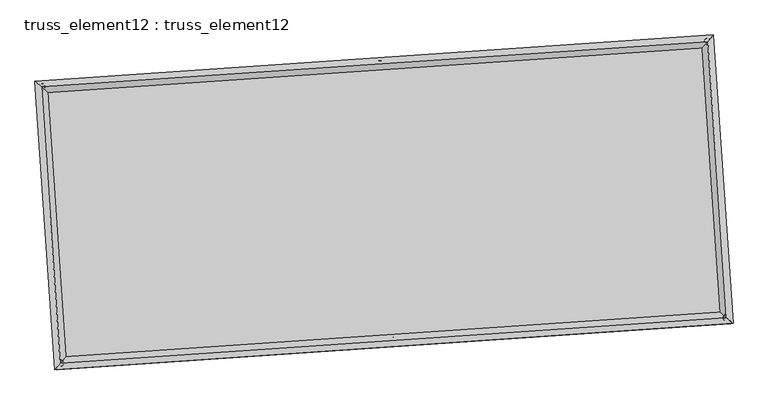
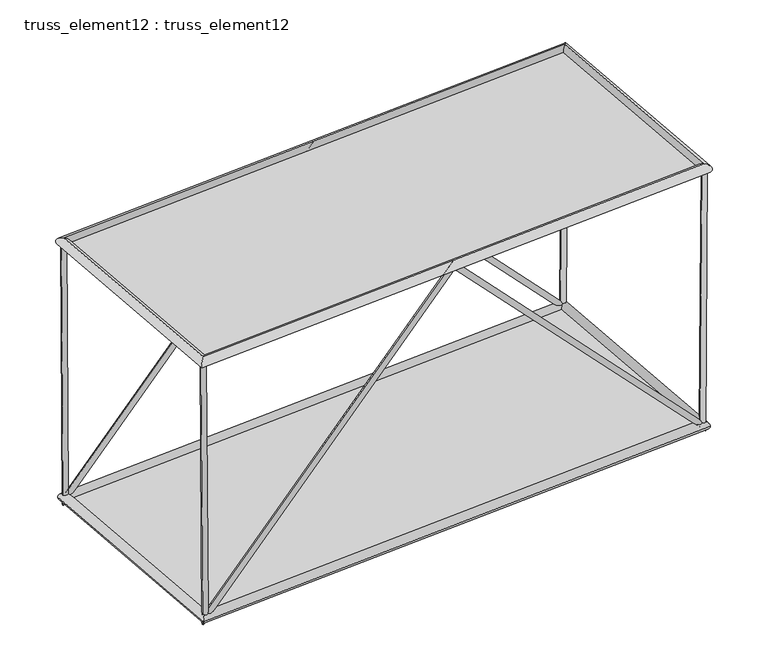
"""IFC4 building model written with IfcOpenShell, lengths in millimetres: plate geometry, truss_element12 : truss_element12."""

from ifc_helpers import new_model, si_unit, frame, origin, origin_with_axes, place, context, project, spatial, polyline, circle_curve, ellipse_curve, outline, extrude, source, transform, mapped, element, save
from ifc_brep_helpers import plane_surface, cylinder_surface, advanced_brep


def truss_element12_truss_element12_8e9da1f8(model_context):
    return source(origin(), model_context, "Body", "SolidModel", [
        advanced_brep(
        [(-3698.7518615, 2273.9185866, 5000.223301), (-3797.8529392, 2260.5574847, 4999.5470243), (-3665.7745625, 2276.1671833, 123.3293266), (-3763.2123204, 2262.9194968, -123.3293266), (1063.9844604, 2598.6714715, 5072.0064402), (1064.4287053, 2592.0979868, 4927.7602832), (5793.2263236, 2921.1404966, 123.3255902), (5891.5346534, 2921.2399919, -123.3255902), (5826.7168605, 2923.424089, 5000.224961), (5926.7142716, 2923.6387563, 4999.5381605)],
        [
            (0, 1, circle_curve(frame((-3748.3024003, 2267.2380357, 4999.8851627), z_axis=(-0.0067617917796413095, -0.00046106087747684727, 0.9999770325336459), x_axis=(-0.13361106793445865, 0.9910337446995272, -0.0004465335886331621)), 50.0)),
            (1, 0, circle_curve(frame((-3748.3024003, 2267.2380357, 4999.8851627), z_axis=(-0.0067617917796413095, -0.00046106087747684727, 0.9999770325336459), x_axis=(-0.13361106793445865, 0.9910337446995272, -0.0004465335886331621)), 50.0)),
            (0, 2),
            (2, 3, ellipse_curve(frame((-3714.4934414, 2269.54334, 0.0), z_axis=(-0.9270371329382548, -0.06321113809700207, 0.3696031739231987), x_axis=(0.3687469497597502, 0.025143452765731104, 0.9291896974385251)), 133.0168379, 50.0)),
            (3, 1),
            (3, 2, ellipse_curve(frame((-3714.4934414, 2269.54334, 0.0), z_axis=(-0.9270371329382548, -0.06321113809700207, 0.3696031739231987), x_axis=(0.3687469497597502, 0.025143452765731104, 0.9291896974385251)), 133.0168379, 50.0)),
            (2, 4),
            (4, 5, ellipse_curve(frame((1064.2065829, 2595.3847292, 4999.8833617), z_axis=(-0.9976833956976204, -0.06802823820297674, 2.7500260085138387e-05), x_axis=(-2.74365528747556e-05, -1.8707942443931063e-06, -0.9999999996218679)), 72.2801261, 50.0)),
            (5, 3),
            (5, 4, ellipse_curve(frame((1064.2065829, 2595.3847292, 4999.8833617), z_axis=(-0.9976833956976204, -0.06802823820297674, 2.7500260085138387e-05), x_axis=(-2.74365528747556e-05, -1.8707942443931063e-06, -0.9999999996218679)), 72.2801261, 50.0)),
            (4, 6),
            (6, 7, ellipse_curve(frame((5842.3804885, 2921.1902443, 0.0), z_axis=(-0.9270667165570741, -0.0632131552915117, -0.3695286187160294), x_axis=(-0.3686725672674666, -0.0251383809063366, 0.9292193497500056)), 133.0085635, 50.0)),
            (7, 5),
            (7, 6, ellipse_curve(frame((5842.3804885, 2921.1902443, 0.0), z_axis=(-0.9270667165570741, -0.0632131552915117, -0.3695286187160294), x_axis=(-0.3686725672674666, -0.0251383809063366, 0.9292193497500056)), 133.0085635, 50.0)),
            (8, 9, circle_curve(frame((5876.715566, 2923.5314227, 4999.8815607), z_axis=(0.0068670155092968675, 0.0004682356836093084, 0.9999763121461127), x_axis=(-0.00214983747870396, 0.9999975862733836, -0.0004534823281307776)), 50.0)),
            (9, 8, circle_curve(frame((5876.715566, 2923.5314227, 4999.8815607), z_axis=(0.0068670155092968675, 0.0004682356836093084, 0.9999763121461127), x_axis=(-0.00214983747870396, 0.9999975862733836, -0.0004534823281307776)), 50.0)),
            (6, 8),
            (9, 7),
        ],
        [
            plane_surface(frame((-3748.3024003, 2317.2380303, 4999.9082162), z_axis=(-0.006761791779640632, -0.0004610608774721699, 0.9999770325336457), x_axis=(0.9999771388246477, -3.1176689248013658e-06, 0.006761791060906577))),
            cylinder_surface(frame((-3748.3024003, 2267.2380357, 4999.8851627), z_axis=(-0.006761791779641308, -0.00046106087747684716, 0.9999770325336457), x_axis=(-0.13361106793445865, 0.9910337446995272, -0.0004465335886331621)), 50.0),
            cylinder_surface(frame((-3714.4934414, 2269.54334, 0.0), z_axis=(-0.6901703766804573, -0.0470600944026198, -0.7221150868577476), x_axis=(-0.020414252830953418, 0.9987522052200565, -0.045577306298510874)), 50.0),
            cylinder_surface(frame((1064.2065829, 2595.3847292, 4999.8833617), z_axis=(-0.6901307509390454, -0.04705739247394453, 0.7221531336370857), x_axis=(-0.11534910612614199, 0.9922789584550205, -0.045574689503274965)), 50.0),
            plane_surface(frame((5876.715566, 2873.5314282, 4999.9049731), z_axis=(0.006867015509297537, 0.00046823568361033024, 0.9999763121461126), x_axis=(0.9999764217710311, -3.215457516247967e-06, -0.006867014756483772))),
            cylinder_surface(frame((5842.3804885, 2921.1902443, 0.0), z_axis=(-0.0068670155092968675, -0.0004682356836093084, -0.9999763121461127), x_axis=(-0.00214983747870396, 0.9999975862733836, -0.0004534823281307776)), 50.0),
        ],
        [
            (0, [[1, 2]]),
            (1, [[-1, 3, 4, 5]]),
            (1, [[-2, -5, 6, -3]]),
            (2, [[-4, 7, 8, 9]]),
            (2, [[-6, -9, 10, -7]]),
            (3, [[-8, 11, 12, 13]]),
            (3, [[-10, -13, 14, -11]]),
            (4, [[15, 16]]),
            (5, [[-12, 17, -16, 18]]),
            (5, [[-14, -18, -15, -17]]),
        ],
    ),
        advanced_brep(
        [(-3426.6389085, -1716.8149977, 5000.223301), (-3525.7399863, -1730.1760996, 4999.5470243), (-3393.6616095, -1714.566401, 123.3293266), (-3491.0993675, -1727.8140875, -123.3293266), (1336.0974133, -1392.0621128, 5072.0064402), (1336.5416582, -1398.6355975, 4927.7602832), (6065.3392765, -1069.5930877, 123.3255902), (6163.6476063, -1069.4935924, -123.3255902), (6098.8298134, -1067.3094953, 5000.224961), (6198.8272245, -1067.094828, 4999.5381605)],
        [
            (0, 1, circle_curve(frame((-3476.1894474, -1723.4955486, 4999.8851627), z_axis=(-0.006761791779640981, -0.00046106087747676796, 0.9999770325336458), x_axis=(-0.13361106793445865, 0.9910337446995272, -0.0004465335886331968)), 50.0)),
            (1, 0, circle_curve(frame((-3476.1894474, -1723.4955486, 4999.8851627), z_axis=(-0.006761791779640981, -0.00046106087747676796, 0.9999770325336458), x_axis=(-0.13361106793445865, 0.9910337446995272, -0.0004465335886331968)), 50.0)),
            (0, 2),
            (2, 3, ellipse_curve(frame((-3442.3804885, -1721.1902443, 0.0), z_axis=(-0.9270371329382548, -0.06321113809700199, 0.3696031739231986), x_axis=(0.3687469497597501, 0.025143452765731125, 0.9291896974385251)), 133.0168379, 50.0)),
            (3, 1),
            (3, 2, ellipse_curve(frame((-3442.3804885, -1721.1902443, 0.0), z_axis=(-0.9270371329382548, -0.06321113809700199, 0.3696031739231986), x_axis=(0.3687469497597501, 0.025143452765731125, 0.9291896974385251)), 133.0168379, 50.0)),
            (2, 4),
            (4, 5, ellipse_curve(frame((1336.3195358, -1395.3488551, 4999.8833617), z_axis=(-0.9976833956976204, -0.0680282382029767, 2.7500260084977895e-05), x_axis=(-2.7436552874601853e-05, -1.8707942444027149e-06, -0.9999999996218678)), 72.2801261, 50.0)),
            (5, 3),
            (5, 4, ellipse_curve(frame((1336.3195358, -1395.3488551, 4999.8833617), z_axis=(-0.9976833956976204, -0.0680282382029767, 2.7500260084977895e-05), x_axis=(-2.7436552874601853e-05, -1.8707942444027149e-06, -0.9999999996218678)), 72.2801261, 50.0)),
            (4, 6),
            (6, 7, ellipse_curve(frame((6114.4934414, -1069.54334, 0.0), z_axis=(-0.9270667165570744, -0.06321315529151138, -0.3695286187160292), x_axis=(-0.36867256726746617, -0.025138380906336657, 0.9292193497500058)), 133.0085635, 50.0)),
            (7, 5),
            (7, 6, ellipse_curve(frame((6114.4934414, -1069.54334, 0.0), z_axis=(-0.9270667165570744, -0.06321315529151138, -0.3695286187160292), x_axis=(-0.36867256726746617, -0.025138380906336657, 0.9292193497500058)), 133.0085635, 50.0)),
            (8, 9, circle_curve(frame((6148.828519, -1067.2021616, 4999.8815607), z_axis=(0.0068670155092972595, 0.00046823568360912634, 0.9999763121461127), x_axis=(-0.0021498374787036058, 0.9999975862733835, -0.0004534823281305971)), 50.0)),
            (9, 8, circle_curve(frame((6148.828519, -1067.2021616, 4999.8815607), z_axis=(0.0068670155092972595, 0.00046823568360912634, 0.9999763121461127), x_axis=(-0.0021498374787036058, 0.9999975862733835, -0.0004534823281305971)), 50.0)),
            (6, 8),
            (9, 7),
        ],
        [
            plane_surface(frame((-3476.1894474, -1673.495554, 4999.9082162), z_axis=(-0.006761791779640632, -0.00046106087747216866, 0.9999770325336457), x_axis=(0.9999771388246477, -3.1176689248013658e-06, 0.006761791060906577))),
            cylinder_surface(frame((-3476.1894474, -1723.4955486, 4999.8851627), z_axis=(-0.006761791779640981, -0.00046106087747676796, 0.9999770325336458), x_axis=(-0.13361106793445865, 0.9910337446995272, -0.0004465335886331968)), 50.0),
            cylinder_surface(frame((-3442.3804885, -1721.1902443, 0.0), z_axis=(-0.6901703766804571, -0.047060094402619775, -0.7221150868577478), x_axis=(-0.020414252830953338, 0.9987522052200565, -0.04557730629851091)), 50.0),
            cylinder_surface(frame((1336.3195358, -1395.3488551, 4999.8833617), z_axis=(-0.6901307509390455, -0.04705739247394449, 0.7221531336370857), x_axis=(-0.11534910612614203, 0.9922789584550205, -0.04557468950327508)), 50.0),
            plane_surface(frame((6148.828519, -1117.2021561, 4999.9049731), z_axis=(0.006867015509297537, 0.0004682356836103296, 0.9999763121461126), x_axis=(0.9999764217710311, -3.215457516247967e-06, -0.006867014756483772))),
            cylinder_surface(frame((6114.4934414, -1069.54334, 0.0), z_axis=(-0.0068670155092972595, -0.00046823568360912634, -0.9999763121461127), x_axis=(-0.0021498374787036058, 0.9999975862733835, -0.0004534823281305971)), 50.0),
        ],
        [
            (0, [[1, 2]]),
            (1, [[-1, 3, 4, 5]]),
            (1, [[-2, -5, 6, -3]]),
            (2, [[-4, 7, 8, 9]]),
            (2, [[-6, -9, 10, -7]]),
            (3, [[-8, 11, 12, 13]]),
            (3, [[-10, -13, 14, -11]]),
            (4, [[15, 16]]),
            (5, [[-12, 17, -16, 18]]),
            (5, [[-14, -18, -15, -17]]),
        ],
    ),
        advanced_brep(
        [(-3476.1903983, -1723.4966025, 4909.8851627), (-3476.1884965, -1723.4944948, 5089.8851627), (-3748.3013152, 2267.2371206, 5089.8851627), (-3748.3034854, 2267.2389507, 4909.8851627), (5876.7146822, 2923.5303734, 5089.8815607), (5876.7164499, 2923.532472, 4909.8815607), (6148.8275009, -1067.201242, 5089.8815607), (6148.829537, -1067.2030813, 4909.8815607)],
        [
            (0, 1, ellipse_curve(frame((-3476.1894474, -1723.4955486, 4999.8851627), z_axis=(-0.753571923405407, 0.657365466278086, 2.6400514504974096e-07), x_axis=(-0.6573654662780334, -0.7535719234054531, 2.640051450497678e-07)), 127.2792206, 90.0)),
            (1, 2),
            (2, 3, ellipse_curve(frame((-3748.3024003, 2267.2380357, 4999.8851627), z_axis=(-0.6573654662780334, -0.7535719234054531, 2.640051450497922e-07), x_axis=(0.7535719234054074, -0.657365466278086, -2.6400514504976537e-07)), 127.2792206, 90.0)),
            (3, 0),
            (1, 0, ellipse_curve(frame((-3476.1894474, -1723.4955486, 4999.8851627), z_axis=(-0.753571923405407, 0.657365466278086, 2.6400514504974096e-07), x_axis=(-0.6573654662780334, -0.7535719234054531, 2.640051450497678e-07)), 127.2792206, 90.0)),
            (3, 2, ellipse_curve(frame((-3748.3024003, 2267.2380357, 4999.8851627), z_axis=(-0.6573654662780334, -0.7535719234054531, 2.640051450497922e-07), x_axis=(0.7535719234054074, -0.657365466278086, -2.6400514504976537e-07)), 127.2792206, 90.0)),
            (2, 4),
            (4, 5, ellipse_curve(frame((5876.715566, 2923.5314227, 4999.8815607), z_axis=(-0.7535719234054071, 0.6573654662780859, 2.6400514504978967e-07), x_axis=(-0.6573654662780337, -0.7535719234054528, 2.64005145049768e-07)), 127.2792206, 90.0)),
            (5, 3),
            (5, 4, ellipse_curve(frame((5876.715566, 2923.5314227, 4999.8815607), z_axis=(-0.7535719234054071, 0.6573654662780859, 2.6400514504978967e-07), x_axis=(-0.6573654662780337, -0.7535719234054528, 2.64005145049768e-07)), 127.2792206, 90.0)),
            (4, 6),
            (6, 7, ellipse_curve(frame((6148.828519, -1067.2021616, 4999.8815607), z_axis=(0.6573654662780337, 0.7535719234054529, -2.640051450497436e-07), x_axis=(-0.753571923405407, 0.6573654662780861, 2.640051450497652e-07)), 127.2792206, 90.0)),
            (7, 5),
            (7, 6, ellipse_curve(frame((6148.828519, -1067.2021616, 4999.8815607), z_axis=(0.6573654662780337, 0.7535719234054529, -2.640051450497436e-07), x_axis=(-0.753571923405407, 0.6573654662780861, 2.640051450497652e-07)), 127.2792206, 90.0)),
            (6, 1),
            (0, 7),
        ],
        [
            cylinder_surface(frame((-3476.1894474, -1723.4955486, 4999.8851627), z_axis=(0.06802823822870037, -0.9976833960748768, 0.0), x_axis=(-0.997683396010759, -0.06802823822432842, 1.1337253567217425e-05)), 90.0),
            cylinder_surface(frame((-3748.3024003, 2267.2380357, 4999.8851627), z_axis=(-0.9976833960748074, -0.06802823822869285, 3.733596566656734e-07), x_axis=(-0.06802823822052487, 0.9976833960151911, 1.0963893910574207e-05)), 90.0),
            cylinder_surface(frame((5876.715566, 2923.5314227, 4999.8815607), z_axis=(-0.06802823822870019, 0.9976833960748768, 0.0), x_axis=(0.997683396018927, 0.06802823822488518, 1.0590534253930997e-05)), 90.0),
            cylinder_surface(frame((6148.828519, -1067.2021616, 4999.8815607), z_axis=(0.9976833960748073, 0.06802823822869236, -3.733596566656388e-07), x_axis=(0.06802823822869236, -0.9976833960146341, 1.0963893910574209e-05)), 90.0),
        ],
        [
            (0, [[1, 2, 3, 4]]),
            (0, [[5, -4, 6, -2]]),
            (1, [[-3, 7, 8, 9]]),
            (1, [[-6, -9, 10, -7]]),
            (2, [[-8, 11, 12, 13]]),
            (2, [[-10, -13, 14, -11]]),
            (3, [[-12, 15, -1, 16]]),
            (3, [[-14, -16, -5, -15]]),
        ],
    ),
        advanced_brep(
        [(-3358.7115243, -1625.2761972, 0.0), (-3526.0494527, -1817.1042913, 0.0), (-3810.4074885, 2353.2123043, 0.0), (-3618.5793943, 2185.8743758, 0.0), (5926.0494527, 3017.1042913, 0.0), (5758.7115243, 2825.2761972, 0.0), (6210.4074885, -1153.2123043, 0.0), (6018.5793943, -985.8743758, 0.0)],
        [
            (0, 1, ellipse_curve(frame((-3442.3804885, -1721.1902443, 0.0), z_axis=(-0.7535719234054583, 0.6573654662780805, 0.0), x_axis=(-0.6573654662780805, -0.7535719234054583, 0.0)), 127.2792206, 90.0)),
            (1, 2),
            (2, 3, ellipse_curve(frame((-3714.4934414, 2269.54334, 0.0), z_axis=(-0.6573654662780805, -0.7535719234054583, 0.0), x_axis=(0.7535719234054583, -0.6573654662780805, 0.0)), 127.2792206, 90.0)),
            (3, 0),
            (1, 0, ellipse_curve(frame((-3442.3804885, -1721.1902443, 0.0), z_axis=(-0.7535719234054583, 0.6573654662780805, 0.0), x_axis=(-0.6573654662780805, -0.7535719234054583, 0.0)), 127.2792206, 90.0)),
            (3, 2, ellipse_curve(frame((-3714.4934414, 2269.54334, 0.0), z_axis=(-0.6573654662780805, -0.7535719234054583, 0.0), x_axis=(0.7535719234054583, -0.6573654662780805, 0.0)), 127.2792206, 90.0)),
            (2, 4),
            (4, 5, ellipse_curve(frame((5842.3804885, 2921.1902443, 0.0), z_axis=(-0.7535719234054583, 0.6573654662780805, 0.0), x_axis=(-0.6573654662780805, -0.7535719234054583, 0.0)), 127.2792206, 90.0)),
            (5, 3),
            (5, 4, ellipse_curve(frame((5842.3804885, 2921.1902443, 0.0), z_axis=(-0.7535719234054583, 0.6573654662780805, 0.0), x_axis=(-0.6573654662780805, -0.7535719234054583, 0.0)), 127.2792206, 90.0)),
            (4, 6),
            (6, 7, ellipse_curve(frame((6114.4934414, -1069.54334, 0.0), z_axis=(0.6573654662780806, 0.7535719234054583, 0.0), x_axis=(-0.7535719234054584, 0.6573654662780802, 0.0)), 127.2792206, 90.0)),
            (7, 5),
            (7, 6, ellipse_curve(frame((6114.4934414, -1069.54334, 0.0), z_axis=(0.6573654662780806, 0.7535719234054583, 0.0), x_axis=(-0.7535719234054584, 0.6573654662780802, 0.0)), 127.2792206, 90.0)),
            (6, 1),
            (0, 7),
        ],
        [
            cylinder_surface(frame((-3442.3804885, -1721.1902443, 0.0), z_axis=(0.06802823822870305, -0.9976833960748764, 0.0), x_axis=(-0.9976833960748764, -0.06802823822870305, 0.0)), 90.0),
            cylinder_surface(frame((-3714.4934414, 2269.54334, 0.0), z_axis=(-0.9976833960748767, -0.06802823822870038, 0.0), x_axis=(-0.06802823822870038, 0.9976833960748767, 0.0)), 90.0),
            cylinder_surface(frame((5842.3804885, 2921.1902443, 0.0), z_axis=(-0.06802823822870298, 0.9976833960748764, 0.0), x_axis=(0.9976833960748764, 0.06802823822870298, 0.0)), 90.0),
            cylinder_surface(frame((6114.4934414, -1069.54334, 0.0), z_axis=(0.9976833960748767, 0.06802823822870031, 0.0), x_axis=(0.06802823822870031, -0.9976833960748767, 0.0)), 90.0),
        ],
        [
            (0, [[1, 2, 3, 4]]),
            (0, [[5, -4, 6, -2]]),
            (1, [[-3, 7, 8, 9]]),
            (1, [[-6, -9, 10, -7]]),
            (2, [[-8, 11, 12, 13]]),
            (2, [[-10, -13, 14, -11]]),
            (3, [[-12, 15, -1, 16]]),
            (3, [[-14, -16, -5, -15]]),
        ],
    ),
        extrude(outline(polyline([(-3442.3804885, -1721.1902443), (-3714.4934414, 2269.54334), (5842.3804885, 2921.1902443), (6114.4934414, -1069.54334), (-3442.3804885, -1721.1902443)])), origin_with_axes(), (0.0, 0.0, 1.0), 20.0),
        extrude(outline(polyline([(-1999.9999999, 4823.6835474), (2000.0000001, 4823.6835474), (2000.0, -4823.6835474), (-2000.0, -4823.6835475), (-1999.9999999, 4823.6835474)])), frame((1200.2630593, 600.017937, 4999.8833617), z_axis=(3.724947302195416e-07, 2.5398999668638065e-08, 0.9999999999999303), x_axis=(-0.06802823822870314, 0.9976833960748764, 0.0)), (0.0, 0.0, 1.0), 20.0),
    ])


if __name__ == "__main__":
    model = new_model("IFC4")
    model_context = context("Model", 3, world=origin())
    ifc_project = project(units=[si_unit("LENGTHUNIT", "METRE", prefix="MILLI")], contexts=[model_context])
    site = spatial("IfcSite", under=ifc_project)
    building = spatial("IfcBuilding", under=site)
    placement = place(None, origin())
    truss_element12_truss_element12_shape = truss_element12_truss_element12_8e9da1f8(model_context)
    element("IfcPlate", 1, ObjectType="truss_element12 : truss_element12", at=placement, inside=building, context=model_context, shape_type="MappedRepresentation", body=[
        mapped(truss_element12_truss_element12_shape, transform((0.0, 0.0, 0.0), x_axis=(1.0, 0.0, 0.0), y_axis=(0.0, 1.0, 0.0), z_axis=(0.0, 0.0, 1.0))),
    ])
    save(model, "model.ifc")

# Revit data of these elements
# Type "truss_element12 : truss_element12"
#   steellbar1 = 90 mm
#   steelbar2 = 50 mm
#   offset1 = 5000 mm
#   M = Default Roof
# Element 1 (IfcPlate, "truss_element12 : truss_element12")
#   Materials on its faces: "Default Roof"
# Materials
#   "Default Roof": class "Miscellaneous", colour RGB 0 127 0, transparency 0, Comments = "Rendering appearance not upgraded Rendering appearance not upgraded ", Cost = 0
